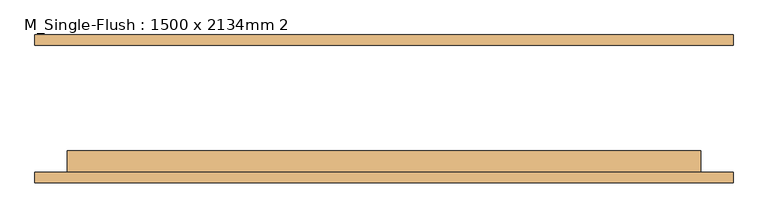
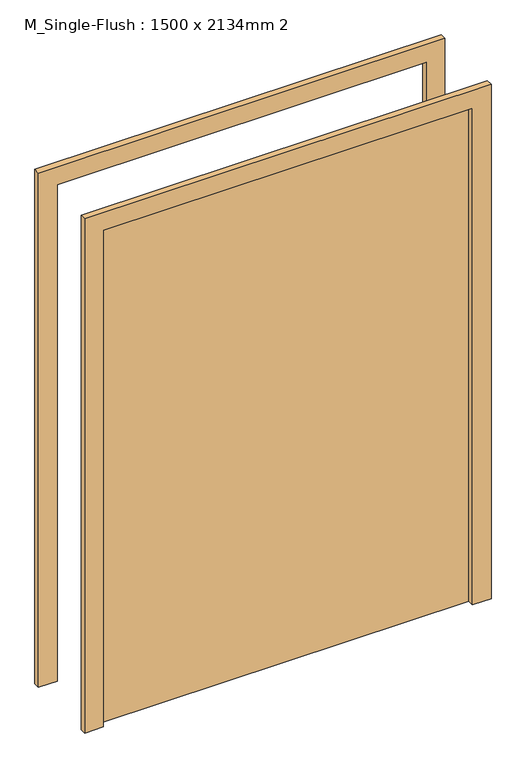
"""IFC4 building model written with IfcOpenShell, lengths in millimetres: door geometry, M_Single-Flush : 1500 x 2134mm 2."""

from ifc_helpers import new_model, si_unit, frame, origin, origin_with_axes, place, context, project, spatial, polyline, outline, extrude, source, transform, mapped, element, save


def m_single_flush_1500_x_2134mm_2_edebd810(model_context):
    return source(origin(), model_context, "Body", "SweptSolid", [
        extrude(outline(polyline([(2210.0, -826.0), (0.0, -826.0), (0.0, -750.0), (2134.0, -750.0), (2134.0, 750.0), (0.0, 750.0), (0.0, 826.0), (2210.0, 826.0), (2210.0, -826.0)])), frame((0.0, -175.0, 0.0), z_axis=(0.0, 1.0, 0.0), x_axis=(0.0, 0.0, 1.0)), (0.0, 0.0, 1.0), 25.0),
        extrude(outline(polyline([(2210.0, 826.0), (2210.0, -826.0), (0.0, -826.0), (0.0, -750.0), (2134.0, -750.0), (2134.0, 750.0), (0.0, 750.0), (0.0, 826.0), (2210.0, 826.0)])), frame((0.0, 150.0, 0.0), z_axis=(0.0, 1.0, 0.0), x_axis=(0.0, 0.0, 1.0)), (0.0, 0.0, 1.0), 25.0),
        extrude(outline(polyline([(750.0, -99.0), (750.0, -150.0), (-750.0, -150.0), (-750.0, -99.0), (750.0, -99.0)])), origin_with_axes(), (0.0, 0.0, 1.0), 2134.0),
    ])


if __name__ == "__main__":
    model = new_model("IFC4")
    model_context = context("Model", 3, world=origin())
    ifc_project = project(units=[si_unit("LENGTHUNIT", "METRE", prefix="MILLI")], contexts=[model_context])
    site = spatial("IfcSite", under=ifc_project)
    building = spatial("IfcBuilding", under=site)
    placement = place(None, origin())
    m_single_flush_1500_x_2134mm_2_shape = m_single_flush_1500_x_2134mm_2_edebd810(model_context)
    element("IfcDoor", 1, ObjectType="M_Single-Flush : 1500 x 2134mm 2", at=placement, inside=building, context=model_context, shape_type="MappedRepresentation", body=[
        mapped(m_single_flush_1500_x_2134mm_2_shape, transform((0.0, 0.0, 0.0), x_axis=(1.0, 0.0, 0.0), y_axis=(0.0, 1.0, 0.0), z_axis=(0.0, 0.0, 1.0))),
    ])
    save(model, "model.ifc")

# Revit data of these elements
# Type "M_Single-Flush : 1500 x 2134mm 2"
#   Type Mark = "34"
#   Thickness = 0.051 m
#   Height = 2.134 m
#   Trim Projection Ext = 0.025 m
#   Trim Projection Int = 0.025 m
#   Trim Width = 0.076 m
#   Width = 1.500 m
#   Door Material = Door - Panel
#   Frame Material = Door - Frame
#   Function = (empty or 0)
#   Wall Closure = (empty or 0)
# Element 1 (IfcDoor, "M_Single-Flush : 1500 x 2134mm 2")
#   Materials on its faces: "Door - Frame", "Door - Panel"
# Materials
#   "Door - Panel": class "Wood", colour RGB 210 159 95, transparency 0
#   "Door - Frame": class "Miscellaneous", colour RGB 118 70 51, transparency 0
